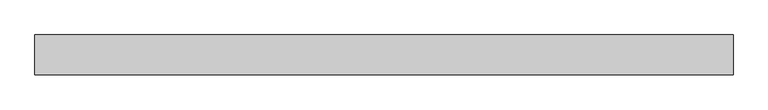
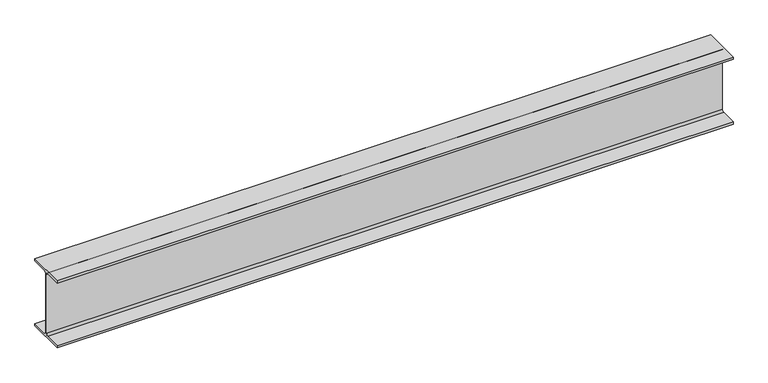
"""IFC4 building model written with IfcOpenShell, lengths in millimetres: beam geometry, Old_Steel Beam_H-KSD3502 : H_SB_ASB_H-250×125x6x9."""

from ifc_helpers import new_model, si_unit, point, frame, frame_2d, origin, place, context, project, spatial, polyline, circle_curve, trimmed, segment, composite_curve, outline, extrude, source, transform, mapped, element, save


def beam_066feed0(model_context):
    return source(origin(), model_context, "Body", "SweptSolid", [
        extrude(outline(composite_curve([segment(polyline([(82.5, -141.5), (82.5, -151.7), (-82.5, -151.7), (-82.5, -141.5), (-11.9, -141.5)]), True, "CONTINUOUS"), segment(trimmed(circle_curve(frame_2d((-11.9, -132.6)), 8.9), [point((-11.9, -141.5))], [point((-3.0, -132.6))], True, "CARTESIAN"), True, "CONTINUOUS"), segment(polyline([(-3.0, -132.6), (-3.0, 132.6)]), True, "CONTINUOUS"), segment(trimmed(circle_curve(frame_2d((-11.9, 132.6)), 8.9), [point((-3.0, 132.6))], [point((-11.9, 141.5))], True, "CARTESIAN"), True, "CONTINUOUS"), segment(polyline([(-11.9, 141.5), (-82.5, 141.5), (-82.5, 151.7), (82.5, 151.7), (82.5, 141.5), (11.9, 141.5)]), True, "CONTINUOUS"), segment(trimmed(circle_curve(frame_2d((11.9, 132.6)), 8.9), [point((11.9, 141.5))], [point((3.0, 132.6))], True, "CARTESIAN"), True, "CONTINUOUS"), segment(polyline([(3.0, 132.6), (3.0, -132.6)]), True, "CONTINUOUS"), segment(trimmed(circle_curve(frame_2d((11.9, -132.6)), 8.9), [point((3.0, -132.6))], [point((11.9, -141.5))], True, "CARTESIAN"), True, "CONTINUOUS"), segment(polyline([(11.9, -141.5), (82.5, -141.5)]), True, "CONTINUOUS")], self_intersect=False)), frame((-1487.2999994, 0.0, 0.0), z_axis=(1.0, 0.0, 0.0), x_axis=(0.0, 1.0, 0.0)), (0.0, 0.0, 1.0), 2892.0999994),
    ])


if __name__ == "__main__":
    model = new_model("IFC4")
    model_context = context("Model", 3, world=origin())
    ifc_project = project(units=[si_unit("LENGTHUNIT", "METRE", prefix="MILLI")], contexts=[model_context])
    site = spatial("IfcSite", under=ifc_project)
    building = spatial("IfcBuilding", under=site)
    placement = place(None, origin())
    beam_shape = beam_066feed0(model_context)
    element("IfcBeam", 1, ObjectType="Old_Steel Beam_H-KSD3502 : H_SB_ASB_H-250×125x6x9", at=placement, inside=building, context=model_context, shape_type="MappedRepresentation", body=[
        mapped(beam_shape, transform((0.0, 0.0, 0.0), x_axis=(1.0, 0.0, 0.0), y_axis=(0.0, 1.0, 0.0), z_axis=(0.0, 0.0, 1.0))),
    ])
    save(model, "model.ifc")

# Revit data of these elements
# Type "Old_Steel Beam_H-KSD3502 : H_SB_ASB_H-250×125x6x9"
#   Width = 12.5 cm
#   Web Thickness = 0.6 cm
#   Web Fillet = 1.2 cm
#   Warping Constant = 42539.8 cm⁶
#   Torsional Moment of Inertia = 7.8102 cm⁴
#   Torsional Modulus = 1.0 cm³
#   Section Area = 37.66 cm²
#   Plastic Modulus weak axis = 73.1 cm³
#   Plastic Modulus strong axis = 366.0 cm³
#   Perimeter = 0.97 m²/m
#   Nominal Weight = 29.60 kgf/m
#   Moment of Inertia weak axis = 294.00 cm⁴
#   Moment of Inertia strong axis = 4050.00 cm⁴
#   Height = 25.0 cm
#   Flange Thickness = 0.9 cm
#   Elastic Modulus weak axis = 47.0 cm³
#   Elastic Modulus strong axis = 324.0 cm³
#   Centroid Vertical = 12.5 cm
#   Centroid Horizontal = 6.25 cm
#   Length [instance default] = 1.5240 m
#   Structural Material [instance default] = Steel, 45-345
#   Assembly Code = ""
# Element 1 (IfcBeam, "Old_Steel Beam_H-KSD3502 : H_SB_ASB_H-250×125x6x9")
#   Structural Material = none
# Materials
#   "Steel, 45-345": class "Metal", colour RGB 189 187 185, transparency 0, Description = "Steel 345 MPa", Cost = 0
